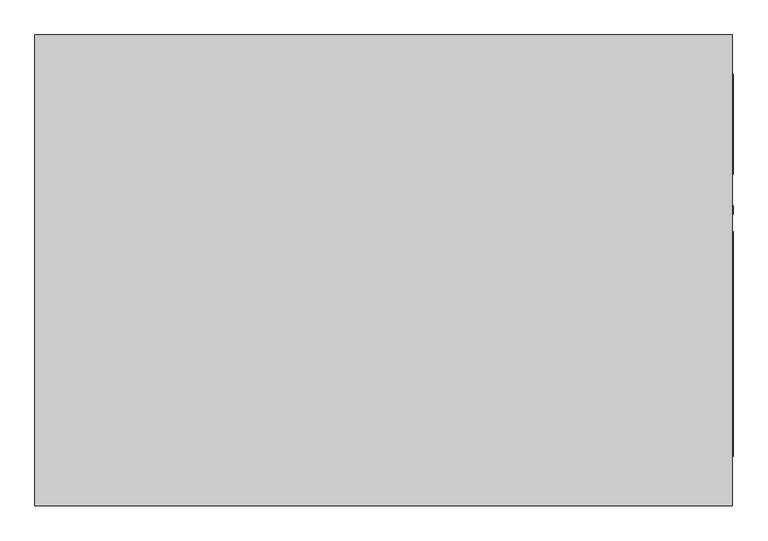
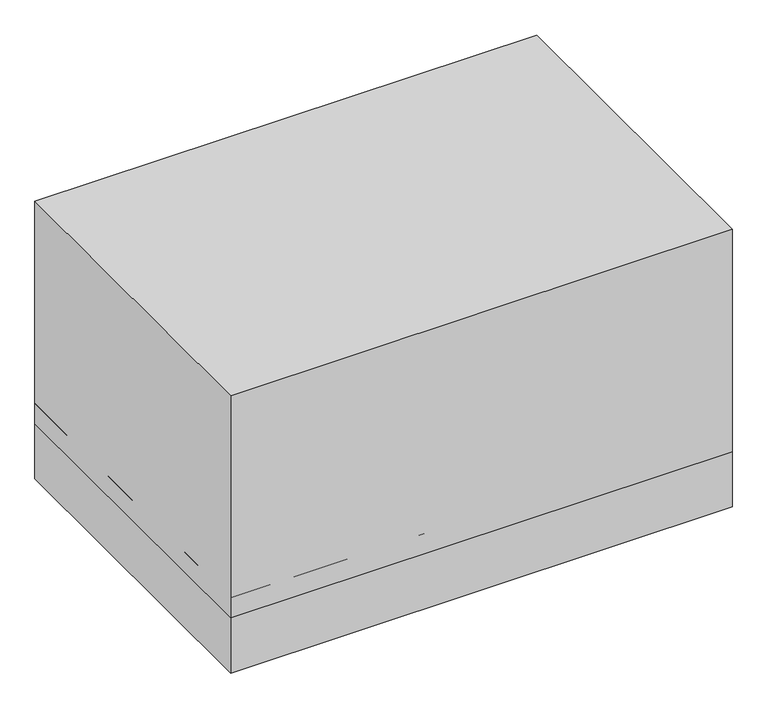
"""IFC4 building model written with IfcOpenShell, lengths in millimetres: proxy geometry, Carrier_48TC_Standard_Efficiency_Gas_Heat_Electric_Cooling_Packaged_Rooftop_Unit_3_to_15_nominal_tons : 7.5 ton 48TC**08."""

from ifc_helpers import new_model, si_unit, point, frame, frame_2d, origin, origin_with_axes, place, context, project, spatial, polyline, circle_curve, trimmed, segment, composite_curve, outline, extrude, source, transform, mapped, element, save
from ifc_brep_helpers import plane_surface, revolved_surface, advanced_brep


def mechanical_equipment_ca1985ec(model_context):
    return source(origin(), model_context, "Body", "SolidModel", [
        extrude(outline(composite_curve([segment(trimmed(circle_curve(frame_2d((193.675, 438.15)), 13.2953125), [point((180.3796875, 438.15))], [point((206.9703125, 438.15))], False, "CARTESIAN"), True, "CONTINUOUS"), segment(trimmed(circle_curve(frame_2d((193.675, 438.15)), 13.2953125), [point((206.9703125, 438.15))], [point((180.3796875, 438.15))], False, "CARTESIAN"), True, "CONTINUOUS")], self_intersect=False)), frame((1119.1875, 0.0, 0.0), z_axis=(1.0, 0.0, 0.0), x_axis=(0.0, 1.0, 0.0)), (0.0, 0.0, 1.0), 3.175),
        advanced_brep(
        [(1119.1875, 755.65, 1308.1), (-1119.1875, 755.65, 1308.1), (-1119.1875, -755.65, 1308.1), (1119.1875, -755.65, 1308.1), (1119.1875, 755.65, 260.35), (1119.1875, -755.65, 260.35), (-1119.1875, -755.65, 260.35), (-1119.1875, 755.65, 260.35), (1036.6375, -596.9, 260.35), (1036.6375, 133.35, 260.35), (681.0375, 133.35, 260.35), (681.0375, -596.9, 260.35), (1036.6375, 590.55, 260.35), (112.7125, 590.55, 260.35), (112.7125, 269.875, 260.35), (1036.6375, 269.875, 260.35), (176.8078125, -107.95, 260.35), (150.2171875, -107.95, 260.35), (-355.6, -476.25, 260.35), (-377.825, -476.25, 260.35), (-344.4875, -349.25, 260.35), (-388.9375, -349.25, 260.35), (-344.4875, -298.45, 260.35), (-388.9375, -298.45, 260.35), (1036.6375, -596.9, 381.0), (681.0375, -596.9, 381.0), (681.0375, 133.35, 381.0), (1036.6375, 133.35, 381.0), (1036.6375, 590.55, 381.0), (1036.6375, 269.875, 381.0), (112.7125, 269.875, 381.0), (112.7125, 590.55, 381.0), (176.8078125, -107.95, 406.4), (150.2171875, -107.95, 406.4), (-355.6, -476.25, 406.4), (-377.825, -476.25, 406.4), (-344.4875, -349.25, 406.4), (-388.9375, -349.25, 406.4), (-344.4875, -298.45, 406.4), (-388.9375, -298.45, 406.4)],
        [
            (0, 1),
            (1, 2),
            (2, 3),
            (3, 0),
            (4, 5),
            (5, 6),
            (6, 7),
            (7, 4),
            (8, 9),
            (9, 10),
            (10, 11),
            (11, 8),
            (12, 13),
            (13, 14),
            (14, 15),
            (15, 12),
            (16, 17, circle_curve(frame((163.5125, -107.95, 260.35), z_axis=(0.0, 0.0, 1.0), x_axis=(-1.0, 0.0, 0.0)), 13.2953125)),
            (17, 16, circle_curve(frame((163.5125, -107.95, 260.35), z_axis=(0.0, 0.0, 1.0), x_axis=(-1.0, 0.0, 0.0)), 13.2953125)),
            (18, 19, circle_curve(frame((-366.7125, -476.25, 260.35), z_axis=(0.0, 0.0, 1.0), x_axis=(-1.0, 0.0, 0.0)), 11.1125)),
            (19, 18, circle_curve(frame((-366.7125, -476.25, 260.35), z_axis=(0.0, 0.0, 1.0), x_axis=(-1.0, 0.0, 0.0)), 11.1125)),
            (20, 21, circle_curve(frame((-366.7125, -349.25, 260.35), z_axis=(0.0, 0.0, 1.0), x_axis=(-1.0, 0.0, 0.0)), 22.225)),
            (21, 20, circle_curve(frame((-366.7125, -349.25, 260.35), z_axis=(0.0, 0.0, 1.0), x_axis=(-1.0, 0.0, 0.0)), 22.225)),
            (22, 23, circle_curve(frame((-366.7125, -298.45, 260.35), z_axis=(0.0, 0.0, 1.0), x_axis=(-1.0, 0.0, 0.0)), 22.225)),
            (23, 22, circle_curve(frame((-366.7125, -298.45, 260.35), z_axis=(0.0, 0.0, 1.0), x_axis=(-1.0, 0.0, 0.0)), 22.225)),
            (0, 4),
            (7, 1),
            (6, 2),
            (5, 3),
            (24, 25),
            (25, 26),
            (26, 27),
            (27, 24),
            (27, 9),
            (8, 24),
            (26, 10),
            (25, 11),
            (28, 29),
            (29, 30),
            (30, 31),
            (31, 28),
            (31, 13),
            (12, 28),
            (30, 14),
            (29, 15),
            (32, 33, circle_curve(frame((163.5125, -107.95, 406.4), z_axis=(0.0, 0.0, -1.0), x_axis=(-1.0, 0.0, 0.0)), 13.2953125)),
            (33, 32, circle_curve(frame((163.5125, -107.95, 406.4), z_axis=(0.0, 0.0, -1.0), x_axis=(-1.0, 0.0, 0.0)), 13.2953125)),
            (33, 17),
            (16, 32),
            (34, 35, circle_curve(frame((-366.7125, -476.25, 406.4), z_axis=(0.0, 0.0, -1.0), x_axis=(-1.0, 0.0, 0.0)), 11.1125)),
            (35, 34, circle_curve(frame((-366.7125, -476.25, 406.4), z_axis=(0.0, 0.0, -1.0), x_axis=(-1.0, 0.0, 0.0)), 11.1125)),
            (35, 19),
            (18, 34),
            (36, 37, circle_curve(frame((-366.7125, -349.25, 406.4), z_axis=(0.0, 0.0, -1.0), x_axis=(-1.0, 0.0, 0.0)), 22.225)),
            (37, 36, circle_curve(frame((-366.7125, -349.25, 406.4), z_axis=(0.0, 0.0, -1.0), x_axis=(-1.0, 0.0, 0.0)), 22.225)),
            (37, 21),
            (20, 36),
            (38, 39, circle_curve(frame((-366.7125, -298.45, 406.4), z_axis=(0.0, 0.0, -1.0), x_axis=(-1.0, 0.0, 0.0)), 22.225)),
            (39, 38, circle_curve(frame((-366.7125, -298.45, 406.4), z_axis=(0.0, 0.0, -1.0), x_axis=(-1.0, 0.0, 0.0)), 22.225)),
            (39, 23),
            (22, 38),
        ],
        [
            plane_surface(frame((-1119.1875, 755.65, 1308.1), z_axis=(0.0, 0.0, 1.0), x_axis=(-1.0, 0.0, 0.0))),
            plane_surface(frame((-1119.1875, 755.65, 260.35), z_axis=(0.0, 0.0, -1.0), x_axis=(1.0, 0.0, 0.0))),
            plane_surface(frame((1119.1875, 755.65, 1308.1), z_axis=(0.0, 1.0, 0.0), x_axis=(0.0, 0.0, -1.0))),
            plane_surface(frame((-1119.1875, 755.65, 1308.1), z_axis=(-1.0, 0.0, 0.0), x_axis=(0.0, 0.0, -1.0))),
            plane_surface(frame((-1119.1875, -755.65, 1308.1), z_axis=(0.0, -1.0, 0.0), x_axis=(0.0, 0.0, -1.0))),
            plane_surface(frame((1119.1875, -755.65, 1308.1), z_axis=(1.0, 0.0, 0.0), x_axis=(0.0, 0.0, -1.0))),
            plane_surface(frame((1036.6375, -596.9, 381.0), z_axis=(0.0, 0.0, -1.0), x_axis=(0.0, 1.0, 0.0))),
            plane_surface(frame((1036.6375, -596.9, 381.0), z_axis=(-1.0, 0.0, 0.0), x_axis=(0.0, 0.0, -1.0))),
            plane_surface(frame((1036.6375, 133.35, 381.0), z_axis=(0.0, -1.0, 0.0), x_axis=(0.0, 0.0, -1.0))),
            plane_surface(frame((681.0375, 133.35, 381.0), z_axis=(1.0, 0.0, 0.0), x_axis=(0.0, 0.0, -1.0))),
            plane_surface(frame((681.0375, -596.9, 381.0), z_axis=(0.0, 1.0, 0.0), x_axis=(0.0, 0.0, -1.0))),
            plane_surface(frame((112.7125, 590.55, 381.0), z_axis=(0.0, 0.0, -1.0), x_axis=(-1.0, 0.0, 0.0))),
            plane_surface(frame((1036.6375, 590.55, 381.0), z_axis=(0.0, -1.0, 0.0), x_axis=(0.0, 0.0, -1.0))),
            plane_surface(frame((112.7125, 590.55, 381.0), z_axis=(1.0, 0.0, 0.0), x_axis=(0.0, 0.0, -1.0))),
            plane_surface(frame((112.7125, 269.875, 381.0), z_axis=(0.0, 1.0, 0.0), x_axis=(0.0, 0.0, -1.0))),
            plane_surface(frame((1036.6375, 269.875, 381.0), z_axis=(-1.0, 0.0, 0.0), x_axis=(0.0, 0.0, -1.0))),
            plane_surface(frame((150.2171875, -107.95, 406.4), z_axis=(0.0, 0.0, -1.0), x_axis=(0.0, -1.0, 0.0))),
            revolved_surface(polyline([(150.2171875, -107.95, 406.4), (150.2171875, -107.95, 260.35)]), (163.5125, -107.95, 0.0), (0.0, 0.0, 1.0)),
            plane_surface(frame((-377.825, -476.25, 406.4), z_axis=(0.0, 0.0, -1.0), x_axis=(0.0, -1.0, 0.0))),
            revolved_surface(polyline([(-377.825, -476.25, 406.4), (-377.825, -476.25, 260.35)]), (-366.7125, -476.25, 0.0), (0.0, 0.0, 1.0)),
            plane_surface(frame((-388.9375, -349.25, 406.4), z_axis=(0.0, 0.0, -1.0), x_axis=(0.0, -1.0, 0.0))),
            revolved_surface(polyline([(-388.9375, -349.25, 406.4), (-388.9375, -349.25, 260.35)]), (-366.7125, -349.25, 0.0), (0.0, 0.0, 1.0)),
            plane_surface(frame((-388.9375, -298.45, 406.4), z_axis=(0.0, 0.0, -1.0), x_axis=(0.0, -1.0, 0.0))),
            revolved_surface(polyline([(-388.9375, -298.45, 406.4), (-388.9375, -298.45, 260.35)]), (-366.7125, -298.45, 0.0), (0.0, 0.0, 1.0)),
        ],
        [
            (0, [[1, 2, 3, 4]]),
            (1, [[5, 6, 7, 8], [9, 10, 11, 12], [13, 14, 15, 16], [17, 18], [19, 20], [21, 22], [23, 24]]),
            (2, [[-1, 25, -8, 26]]),
            (3, [[-2, -26, -7, 27]]),
            (4, [[-3, -27, -6, 28]]),
            (5, [[-4, -28, -5, -25]]),
            (6, [[29, 30, 31, 32]]),
            (7, [[-32, 33, -9, 34]]),
            (8, [[-31, 35, -10, -33]]),
            (9, [[-30, 36, -11, -35]]),
            (10, [[-29, -34, -12, -36]]),
            (11, [[37, 38, 39, 40]]),
            (12, [[-40, 41, -13, 42]]),
            (13, [[-39, 43, -14, -41]]),
            (14, [[-38, 44, -15, -43]]),
            (15, [[-37, -42, -16, -44]]),
            (16, [[45, 46]]),
            (17, [[-46, 47, -17, 48]]),
            (17, [[-45, -48, -18, -47]]),
            (18, [[49, 50]]),
            (19, [[-50, 51, -19, 52]]),
            (19, [[-49, -52, -20, -51]]),
            (20, [[53, 54]]),
            (21, [[-54, 55, -21, 56]]),
            (21, [[-53, -56, -22, -55]]),
            (22, [[57, 58]]),
            (23, [[-58, 59, -23, 60]]),
            (23, [[-57, -60, -24, -59]]),
        ],
    ),
        extrude(outline(polyline([(1119.1875, 755.65), (1119.1875, -755.65), (-1119.1875, -755.65), (-1119.1875, 755.65), (1119.1875, 755.65)]), holes=[polyline([(1036.6375, 590.55), (112.7125, 590.55), (112.7125, 269.875), (1036.6375, 269.875), (1036.6375, 590.55)]), polyline([(1036.6375, -596.9), (1036.6375, 133.35), (681.0375, 133.35), (681.0375, -596.9), (1036.6375, -596.9)]), composite_curve([segment(trimmed(circle_curve(frame_2d((163.5125, -107.95)), 13.2953125), [point((176.8078125, -107.95))], [point((150.2171875, -107.95))], True, "CARTESIAN"), True, "CONTINUOUS"), segment(trimmed(circle_curve(frame_2d((163.5125, -107.95)), 13.2953125), [point((150.2171875, -107.95))], [point((176.8078125, -107.95))], True, "CARTESIAN"), True, "CONTINUOUS")], self_intersect=False), composite_curve([segment(trimmed(circle_curve(frame_2d((-366.7125, -476.25)), 11.1125), [point((-355.6, -476.25))], [point((-377.825, -476.25))], True, "CARTESIAN"), True, "CONTINUOUS"), segment(trimmed(circle_curve(frame_2d((-366.7125, -476.25)), 11.1125), [point((-377.825, -476.25))], [point((-355.6, -476.25))], True, "CARTESIAN"), True, "CONTINUOUS")], self_intersect=False), composite_curve([segment(trimmed(circle_curve(frame_2d((-366.7125, -349.25)), 22.225), [point((-344.4875, -349.25))], [point((-388.9375, -349.25))], True, "CARTESIAN"), True, "CONTINUOUS"), segment(trimmed(circle_curve(frame_2d((-366.7125, -349.25)), 22.225), [point((-388.9375, -349.25))], [point((-344.4875, -349.25))], True, "CARTESIAN"), True, "CONTINUOUS")], self_intersect=False), composite_curve([segment(trimmed(circle_curve(frame_2d((-366.7125, -298.45)), 22.225), [point((-344.4875, -298.45))], [point((-388.9375, -298.45))], True, "CARTESIAN"), True, "CONTINUOUS"), segment(trimmed(circle_curve(frame_2d((-366.7125, -298.45)), 22.225), [point((-388.9375, -298.45))], [point((-344.4875, -298.45))], True, "CARTESIAN"), True, "CONTINUOUS")], self_intersect=False)]), origin_with_axes(), (0.0, 0.0, 1.0), 355.6),
        extrude(outline(polyline([(1122.3625, 628.65), (1122.3625, 307.975), (1119.1875, 307.975), (1119.1875, 628.65), (1122.3625, 628.65)])), frame((0.0, 0.0, 406.4), z_axis=(0.0, 0.0, 1.0), x_axis=(1.0, 0.0, 0.0)), (0.0, 0.0, 1.0), 857.25),
        extrude(outline(polyline([(1122.3625, 123.825), (1122.3625, -596.9), (1119.1875, -596.9), (1119.1875, 123.825), (1122.3625, 123.825)])), frame((0.0, 0.0, 406.4), z_axis=(0.0, 0.0, 1.0), x_axis=(1.0, 0.0, 0.0)), (0.0, 0.0, 1.0), 352.425),
    ])


if __name__ == "__main__":
    model = new_model("IFC4")
    model_context = context("Model", 3, world=origin())
    ifc_project = project(units=[si_unit("LENGTHUNIT", "METRE", prefix="MILLI")], contexts=[model_context])
    site = spatial("IfcSite", under=ifc_project)
    building = spatial("IfcBuilding", under=site)
    placement = place(None, origin())
    mechanical_equipment_shape = mechanical_equipment_ca1985ec(model_context)
    element("IfcBuildingElementProxy", 1, Name="Carrier_48TC_Standard_Efficiency_Gas_Heat_Electric_Cooling_Packaged_Rooftop_Unit_3_to_15_nominal_tons : 7.5 ton 48TC**08", ObjectType="Carrier_48TC_Standard_Efficiency_Gas_Heat_Electric_Cooling_Packaged_Rooftop_Unit_3_to_15_nominal_tons : 7.5 ton 48TC**08", at=placement, inside=building, context=model_context, shape_type="MappedRepresentation", body=[
        mapped(mechanical_equipment_shape, transform((0.0, 0.0, 0.0), x_axis=(1.0, 0.0, 0.0), y_axis=(0.0, 1.0, 0.0), z_axis=(0.0, 0.0, 1.0))),
    ])
    save(model, "model.ifc")

# Revit data of these elements
# Type "Carrier_48TC_Standard_Efficiency_Gas_Heat_Electric_Cooling_Packaged_Rooftop_Unit_3_to_15_nominal_tons : 7.5 ton 48TC**08"
#   URL = "www.Carrier.com"
#   Model = "48TC"
#   Manufacturer = "Carrier"
#   Disclaimer = "Manufacturer reserves the right to change, at any time, specifications and designs without notice and without obligation.  Please verify critical parameters with local Carrier commercial sales office."
#   knockout thickness = 0' - 0 1/16"
#   Voltage = 0 V
#   Version = 1
#   TTBY3 = 0' - 11"
#   TTBY2 = 1' - 4"
#   TTBY1 = 1' - 6"
#   TTBX = 2' - 5 5/8"
#   TTBPowerR = 0' - 0 7/8"
#   TTBGasR = 0' - 0 7/8"
#   SSSZ = 0' - 5 3/4"
#   SSSY = 0' - 6 1/4"
#   SSSW = 2' - 4 3/8"
#   SSSH = 1' - 1 7/8"
#   SSRZ = 0' - 5 3/4"
#   SSRY = 0' - 5"
#   SSRW = 1' - 0 5/8"
#   SSRH = 2' - 9 3/4"
#   SEER = 0
#   Right clearance = 3' - 0"
#   PWRZ = 2' - 3 7/8"
#   PWRY = 0' - 4 5/8"
#   PWRR = 0' - 1 1/4"
#   ODF2X = 1' - 0"
#   ODF1Y = 0' - 11"
#   ODF1X = 2' - 1"
#   ODF1R = 0' - 10"
#   MOCP = 0 A
#   MCA = 0 A
#   Left clearance = 4' - 0"
#   IEER = 11.7
#   Front clearance = 4' - 0"
#   Fan Z = 4' - 3 1/2"
#   Width = 4' - 11 1/2"
#   Length = 7' - 4 1/8"
#   Height = 3' - 5 1/4"
#   EER = 11
#   DSSY = 0' - 6 1/4"
#   DSSX = 0' - 3 1/4"
#   DSSW = 1' - 2"
#   DSSH = 2' - 4 3/4"
#   DSRY = 0' - 6 1/2"
#   DSRX = 0' - 3 1/4"
#   DSRW = 3' - 0 3/8"
#   DSRH = 1' - 0 5/8"
#   DRNZ = 0' - 7"
#   DRNY = 3' - 1 3/8"
#   DRNR = 0' - 0 67/128"
#   Curb Z = 1' - 2"
#   CFM (nominal) = 0 CFM
#   Back clearance = 3' - 0"
#   Alt Condensate Drain = 0' - 0 67/128"
#   AccypwrR = 0' - 0 7/16"
#   ACY = 2' - 1 1/2"
#   ACX = 3' - 1 5/8"
#   Gas [instance default] = yes
#   Fan 2 on = yes
#   Curb_1SLAB_2ROOFCURB_3SNOWCURB = 2
#   Fan 3 on = no
#   Unit material = RTU
#   Curb material = Curb paint
# Element 1 (IfcBuildingElementProxy, "Carrier_48TC_Standard_Efficiency_Gas_Heat_Electric_Cooling_Packaged_Rooftop_Unit_3_to_15_nominal_tons : 7.5 ton 48TC**08")
#   Materials on its faces: "RTU", "Curb paint", "Mech"
# Materials
#   "RTU": class "Miscellaneous", colour RGB 104 104 104, transparency 0, Cost = 0
#   "Curb paint": class "Miscellaneous", colour RGB 189 187 185, transparency 0
#   "Mech": class "Miscellaneous", colour RGB 235 237 235, transparency 0, Cost = 0
